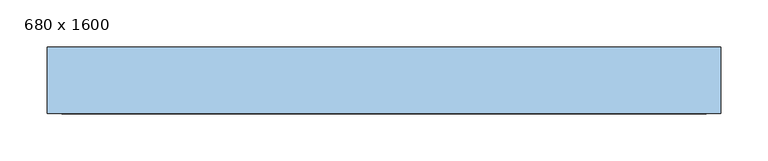
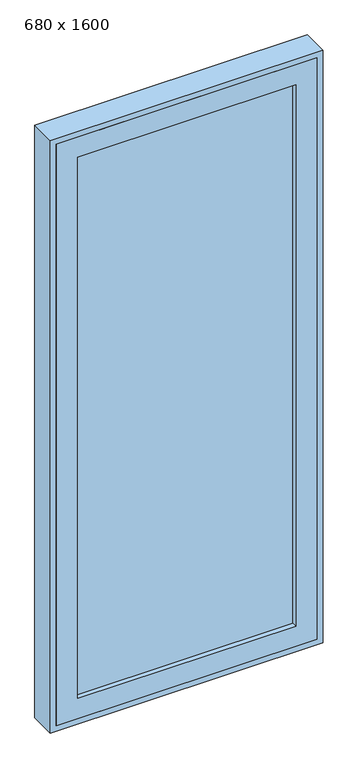
"""IFC4 building model written with IfcOpenShell, lengths in millimetres: window geometry, Aluprof_MB-79N-SI_E_Alu_Window-1sash-FIX_ENG_R-00206 : 680 x 1600."""

import ifcopenshell
import ifcopenshell.guid

model = None  # the IFC model being written
_history = None  # IfcOwnerHistory: only IFC2X3 demands one
_inside = {}  # id of a spatial element -> (the spatial element, [elements in it])
_under = {}  # id of a project, library or spatial element -> (it, [spatial elements below it])
_declared = {}  # id of a project -> (the project, [libraries it declares])
_typed = {}  # id of a type object -> (the type object, [elements of that type])
_made_of = {}  # id of a material, layer set ... -> (it, [elements and type objects made of it])


def new_model(schema):
    """Start an empty IFC model of exactly this schema.

    Asked for "IFC4X3", IfcOpenShell would pick the latest addendum, in which some entities
    have other attributes; the version numbers below select the first issue.
    IFC2X3 requires an IfcOwnerHistory on every rooted entity: one is made here for all.
    """
    global model, _history
    if schema == "IFC4X3":
        model = ifcopenshell.file(schema_version=(4, 3, 0, 0))
    else:
        model = ifcopenshell.file(schema=schema)
    _inside.clear()
    _under.clear()
    _declared.clear()
    _typed.clear()
    _made_of.clear()
    _history = None
    if model.schema == "IFC2X3":
        org = make("IfcOrganization", Name="unknown")
        user = make(
            "IfcPersonAndOrganization",
            ThePerson=make("IfcPerson", FamilyName="unknown"),
            TheOrganization=org,
        )
        app = make(
            "IfcApplication",
            ApplicationDeveloper=org,
            Version="unknown",
            ApplicationFullName="unknown",
            ApplicationIdentifier="unknown",
        )
        _history = make(
            "IfcOwnerHistory",
            OwningUser=user,
            OwningApplication=app,
            ChangeAction="ADDED",
            CreationDate=0,
        )
    return model


def make(cls, **values):
    """One entity of the class cls with the attributes given. An attribute that is None is left unset."""
    return model.create_entity(
        cls, **{name: value for name, value in values.items() if value is not None}
    )


def rooted(cls, **values):
    """An entity with a GlobalId (a new one), such as an element, a storey or a relation."""
    return make(cls, GlobalId=ifcopenshell.guid.new(), OwnerHistory=_history, **values)


def si_unit(unit_type, name, prefix=None):
    """IfcSIUnit, for example si_unit("LENGTHUNIT", "METRE", prefix="MILLI")."""
    return make("IfcSIUnit", UnitType=unit_type, Prefix=prefix, Name=name)


def assignment(units):
    """IfcUnitAssignment: the units of a project."""
    return None if units is None else make("IfcUnitAssignment", Units=units)


def point(xyz):
    """IfcCartesianPoint."""
    return None if xyz is None else make("IfcCartesianPoint", Coordinates=xyz)


def direction(xyz):
    """IfcDirection."""
    return None if xyz is None else make("IfcDirection", DirectionRatios=xyz)


def frame(location, z_axis=None, x_axis=None):
    """IfcAxis2Placement3D, a coordinate frame: its origin and axes. An axis left out is left unset."""
    return make(
        "IfcAxis2Placement3D",
        Location=point(location),
        Axis=direction(z_axis),
        RefDirection=direction(x_axis),
    )


def origin():
    """The frame at (0, 0, 0) with its axes left unset."""
    return frame((0.0, 0.0, 0.0))


def place(relative_to, where):
    """IfcLocalPlacement: puts the frame where relative to a parent placement (None: the world)."""
    return make(
        "IfcLocalPlacement", PlacementRelTo=relative_to, RelativePlacement=where
    )


def context(
    kind, dimensions, precision=None, world=None, true_north=None, identifier=None
):
    """IfcGeometricRepresentationContext, for example the 3D "Model" context."""
    return make(
        "IfcGeometricRepresentationContext",
        ContextIdentifier=identifier,
        ContextType=kind,
        CoordinateSpaceDimension=dimensions,
        Precision=precision,
        WorldCoordinateSystem=world,
        TrueNorth=true_north,
    )


def project(units=None, contexts=None):
    """IfcProject with its units and contexts."""
    return rooted(
        "IfcProject",
        Name="project",
        RepresentationContexts=contexts,
        UnitsInContext=assignment(units),
    )


def spatial(cls, under=None, at=None, **own):
    """A site, building, storey or space (cls), placed at a placement, below another one or the project."""
    s = rooted(cls, ObjectPlacement=at, **own)
    if under is not None:
        _under.setdefault(under.id(), (under, []))[1].append(s)
    return s


def polyline(points):
    """IfcPolyline through the points."""
    return make("IfcPolyline", Points=[point(p) for p in points])


def outline(outer, holes=None, kind="AREA"):
    """IfcArbitraryClosedProfileDef: a profile drawn as a closed curve; with holes, ...WithVoids."""
    if holes is None:
        return make("IfcArbitraryClosedProfileDef", ProfileType=kind, OuterCurve=outer)
    return make(
        "IfcArbitraryProfileDefWithVoids",
        ProfileType=kind,
        OuterCurve=outer,
        InnerCurves=holes,
    )


def extrude(swept, where, along, depth):
    """IfcExtrudedAreaSolid: the profile swept, set in the frame where, extruded along a direction by depth."""
    return make(
        "IfcExtrudedAreaSolid",
        SweptArea=swept,
        Position=where,
        ExtrudedDirection=direction(along),
        Depth=depth,
    )


def faces_of(points, faces, orient=None, outer=None):
    """IfcFace entities. A face is a list of loops; a loop is a list of indices into points, from 0.

    orient and outer hold one flag for each loop. By default every Orientation is true, the
    first loop of a face is its IfcFaceOuterBound and the others are IfcFaceBound.
    """
    made = []
    for i, loops in enumerate(faces):
        bounds = []
        for j, loop in enumerate(loops):
            is_outer = j == 0 if outer is None else outer[i][j]
            bounds.append(
                make(
                    "IfcFaceOuterBound" if is_outer else "IfcFaceBound",
                    Bound=make("IfcPolyLoop", Polygon=[points[k] for k in loop]),
                    Orientation=True if orient is None else orient[i][j],
                )
            )
        made.append(make("IfcFace", Bounds=bounds))
    return made


def faceted_brep(points, faces, orient=None, outer=None, voids=None):
    """IfcFacetedBrep: a solid bounded by flat faces; with voids (closed shells), ...WithVoids."""
    shared = [point(p) for p in points]
    hull = make("IfcClosedShell", CfsFaces=faces_of(shared, faces, orient, outer))
    if voids is None:
        return make("IfcFacetedBrep", Outer=hull)
    return make(
        "IfcFacetedBrepWithVoids",
        Outer=hull,
        Voids=[
            make(cls, CfsFaces=faces_of(shared, fs, o, b)) for cls, fs, o, b in voids
        ],
    )


def shape(context_of_items, identifier, shape_type, items):
    """IfcShapeRepresentation: the items that make up one representation, for example the "Body"."""
    return make(
        "IfcShapeRepresentation",
        ContextOfItems=context_of_items,
        RepresentationIdentifier=identifier,
        RepresentationType=shape_type,
        Items=items,
    )


def source(mapping_origin, context_of_items, identifier, shape_type, items):
    """IfcRepresentationMap: a shape defined once, which mapped items show again and again."""
    return make(
        "IfcRepresentationMap",
        MappingOrigin=mapping_origin,
        MappedRepresentation=shape(context_of_items, identifier, shape_type, items),
    )


def transform(
    local_origin,
    x_axis=None,
    y_axis=None,
    z_axis=None,
    scale=None,
    scale2=None,
    scale3=None,
    uniform=True,
):
    """IfcCartesianTransformationOperator3D, or its non-uniform kind. x_axis, y_axis, z_axis: its Axis1, 2, 3."""
    if uniform:
        return make(
            "IfcCartesianTransformationOperator3D",
            Axis1=direction(x_axis),
            Axis2=direction(y_axis),
            LocalOrigin=point(local_origin),
            Scale=scale,
            Axis3=direction(z_axis),
        )
    return make(
        "IfcCartesianTransformationOperator3DnonUniform",
        Axis1=direction(x_axis),
        Axis2=direction(y_axis),
        LocalOrigin=point(local_origin),
        Scale=scale,
        Axis3=direction(z_axis),
        Scale2=scale2,
        Scale3=scale3,
    )


def mapped(mapping_source, mapping_target):
    """IfcMappedItem: shows the shape of a source again, moved by a transform."""
    return make(
        "IfcMappedItem", MappingSource=mapping_source, MappingTarget=mapping_target
    )


def made_of(thing, what):
    """Note that an element or type object is made of a material, layer set ...; save() writes the relation."""
    if what is not None:
        _made_of.setdefault(what.id(), (what, []))[1].append(thing)
    return thing


def element(
    cls,
    number,
    at=None,
    inside=None,
    cuts=None,
    type_object=None,
    material=None,
    context=None,
    identifier="Body",
    shape_type=None,
    held_by="IfcProductDefinitionShape",
    body=None,
    shapes=None,
    **own,
):
    """One element of the class cls, such as IfcWall. Its Tag is "e" and its number.

    at: its placement. inside: the storey or other place that contains it. cuts: it is an
    opening in that element (IfcRelVoidsElement). A single representation is given by context,
    identifier, shape_type and body (its items); several are given by shapes. held_by: the class
    of the entity that holds the representations. save() writes the other relations.
    """
    e = rooted(cls, Tag="e%d" % number, ObjectPlacement=at, **own)
    if body is not None:
        shapes = [shape(context, identifier, shape_type, body)]
    if shapes is not None:
        e.Representation = make(held_by, Representations=shapes)
    if inside is not None:
        _inside.setdefault(inside.id(), (inside, []))[1].append(e)
    if cuts is not None:
        rooted(
            "IfcRelVoidsElement", RelatingBuildingElement=cuts, RelatedOpeningElement=e
        )
    if type_object is not None:
        _typed.setdefault(type_object.id(), (type_object, []))[1].append(e)
    return made_of(e, material)


def aggregate(whole, parts):
    """IfcRelAggregates: a whole, such as a stair, and the parts it consists of."""
    return rooted("IfcRelAggregates", RelatingObject=whole, RelatedObjects=parts)


def save(model, path):
    """Write the relations noted so far, then the file.

    IfcRelAggregates (storeys below a building ...), IfcRelContainedInSpatialStructure (elements
    in a storey), IfcRelDefinesByType, IfcRelAssociatesMaterial and IfcRelDeclares: one each for
    every whole, place, type object, material and project.
    """
    for whole, parts in _under.values():
        aggregate(whole, parts)
    for where, things in _inside.values():
        rooted(
            "IfcRelContainedInSpatialStructure",
            RelatedElements=things,
            RelatingStructure=where,
        )
    for kind, things in _typed.values():
        rooted("IfcRelDefinesByType", RelatedObjects=things, RelatingType=kind)
    for what, things in _made_of.values():
        rooted("IfcRelAssociatesMaterial", RelatedObjects=things, RelatingMaterial=what)
    for by, libraries in _declared.values():
        rooted("IfcRelDeclares", RelatingContext=by, RelatedDefinitions=libraries)
    model.write(path)


def window_680_x_1600_0a658332(model_context):
    return source(origin(), model_context, "Body", "SolidModel", [
        faceted_brep([(-284.5, 58.5, 2315.5), (-284.5, 45.0, 2315.5), (-284.5, 45.0, 826.5), (-284.5, 58.5, 826.5), (-340.0, 45.0, 2371.0), (-340.0, 115.0, 2371.0), (-340.0, 115.0, 771.0), (-340.0, 45.0, 771.0), (284.5, 45.0, 826.5), (284.5, 58.5, 826.5), (340.0, 115.0, 771.0), (340.0, 45.0, 771.0), (284.5, 45.0, 2315.5), (284.5, 58.5, 2315.5), (340.0, 115.0, 2371.0), (340.0, 45.0, 2371.0), (-300.5, 58.5, 2331.5), (300.5, 58.5, 2331.5), (300.5, 58.5, 810.5), (-300.5, 58.5, 810.5), (-300.5, 106.5, 2331.5), (-300.5, 106.5, 810.5), (300.5, 106.5, 810.5), (300.5, 106.5, 2331.5), (-281.5, 106.5, 2312.5), (281.5, 106.5, 2312.5), (281.5, 106.5, 829.5), (-281.5, 106.5, 829.5), (-281.5, 115.0, 2312.5), (-281.5, 115.0, 829.5), (281.5, 115.0, 829.5), (281.5, 115.0, 2312.5)], [[[0, 1, 2, 3]], [[4, 5, 6, 7]], [[3, 2, 8, 9]], [[7, 6, 10, 11]], [[9, 8, 12, 13]], [[11, 10, 14, 15]], [[16, 17, 18, 19], [3, 9, 13, 0]], [[13, 12, 1, 0]], [[7, 11, 15, 4], [1, 12, 8, 2]], [[15, 14, 5, 4]], [[20, 16, 19, 21]], [[21, 19, 18, 22]], [[22, 18, 17, 23]], [[21, 22, 23, 20], [24, 25, 26, 27]], [[23, 17, 16, 20]], [[28, 24, 27, 29]], [[29, 27, 26, 30]], [[30, 26, 25, 31]], [[5, 14, 10, 6], [29, 30, 31, 28]], [[31, 25, 24, 28]]]),
        extrude(outline(polyline([(300.5, 58.5), (-300.5, 58.5), (-300.5, 106.5), (300.5, 106.5), (300.5, 58.5)])), frame((0.0, 0.0, 810.5), z_axis=(0.0, 0.0, 1.0), x_axis=(1.0, 0.0, 0.0)), (0.0, 0.0, 1.0), 1521.0),
        extrude(outline(polyline([(756.0, -355.0), (756.0, 355.0), (2386.0, 355.0), (2386.0, -355.0), (756.0, -355.0)]), holes=[polyline([(2371.0, -340.0), (2371.0, 340.0), (771.0, 340.0), (771.0, -340.0), (2371.0, -340.0)])]), frame((0.0, 45.0, 0.0), z_axis=(0.0, 1.0, 0.0), x_axis=(0.0, 0.0, 1.0)), (0.0, 0.0, 1.0), 70.0),
    ])


if __name__ == "__main__":
    model = new_model("IFC4")
    model_context = context("Model", 3, world=origin())
    ifc_project = project(units=[si_unit("LENGTHUNIT", "METRE", prefix="MILLI")], contexts=[model_context])
    site = spatial("IfcSite", under=ifc_project)
    building = spatial("IfcBuilding", under=site)
    placement = place(None, origin())
    window_680_x_1600_shape = window_680_x_1600_0a658332(model_context)
    element("IfcWindow", 1, ObjectType="Aluprof_MB-79N-SI_E_Alu_Window-1sash-FIX_ENG_R-00206 : 680 x 1600", at=placement, inside=building, context=model_context, shape_type="MappedRepresentation", body=[
        mapped(window_680_x_1600_shape, transform((0.0, 0.0, 0.0), x_axis=(1.0, 0.0, 0.0), y_axis=(0.0, 1.0, 0.0), z_axis=(0.0, 0.0, 1.0))),
    ])
    save(model, "model.ifc")

# Revit data of these elements
# Type "Aluprof_MB-79N-SI_E_Alu_Window-1sash-FIX_ENG_R-00206 : 680 x 1600"
#   Type Mark = "50"
#   Water resistance = "Class E1950, EN 12208"
#   Uniclass2015Version = "v1.6"
#   Uniclass2015Reference = "Pr_30_59_98_02"
#   Uniclass2015Description = "Aluminium window units"
#   URL = "https://aluprof.eu/"
#   Resistance to wind load = "Class C5, EN 12210"
#   Product page URL = "https://aluprof.eu/architekci/katalog-dla-architektow/systemy-okienno-drzwiowe/mb-79n-si-system-okienno-drzwiowy-z-izolacja-termiczna#/materialy/ogolne-informacje"
#   Operation = "SinglePanel"
#   Opening type = "FIX"
#   NBSReference = "45-25-99/310"
#   NBSDescription = "Aluminium window units"
#   Model = "MB-79N SI"
#   Manufacturer = "ALUPROF S.A."
#   Insert type = "SI"
#   IfcExportType = "NOTDEFINED"
#   IfcExportAs = "IfcWindowType"
#   Glazing construction = "6/16/4/16/6"
#   Description = "Single fixed window"
#   Content of the recyclate in the material = "70.7%"
#   COBie.Type.WarrantyDurationParts = ""
#   COBie.Type.Name = ""
#   COBie.Type.Manufacturer = "ALUPROF SA"
#   COBie.Space.Name = ""
#   COBie.Floor.Name = ""
#   COBie.Facility.Name = ""
#   COBie.CreatedOn = ""
#   COBie.CreatedBy = "aluprof.eu"
#   COBie.Component.WarrantyStartDate = ""
#   COBie.Component.Name = "MB-79N SI"
#   Air permeability = "Class 4, EN 12207"
#   Thermal insulation = 0.6000 W/(m²·K)
#   Sash thickness = 79 mm
#   Rough Width = 710 mm
#   Rough Height = 1630 mm
#   Mounting space = 15 mm
#   Height = 1600 mm
#   Glazing area = 0.914121 m²
#   Frame thickness = 70 mm
#   Exterior wall face offset = 60 mm
#   Sill Height = 771 mm
#   Width = 680 mm
#   Warm installation [instance default] = yes
#   Schedule No. [instance default] = 1
#   IsExternal = yes
#   COBie.Type = yes
#   COBie = yes
#   GlazingMaterial = Glass_ALUPROF_Clear
#   FrameMaterial = Träfönster WSP Stockholm
#   BackfillingMaterial = ExpandingFoam_ALUPROF_Yellow
#   Wall Closure = (empty or 0)
# Element 1 (IfcWindow, "Aluprof_MB-79N-SI_E_Alu_Window-1sash-FIX_ENG_R-00206 : 680 x 1600")
#   Materials on its faces: "Träfönster WSP Stockholm", "ExpandingFoam_ALUPROF_Yellow", "Glass_ALUPROF_Clear"
# Materials
#   "Glass_ALUPROF_Clear": class "Glass", colour RGB 22 81 169, transparency 0.85, Model = "GlazingClear", Manufacturer = "ALUPROF S.A.", URL = "https://aluprof.eu/pl-en", Description = "Glazing", Cost = 0
#   "Träfönster WSP Stockholm": class "Generic", colour RGB 45 25 19, transparency 0, Cost = 0
#   "ExpandingFoam_ALUPROF_Yellow": class "Generic", colour RGB 175 175 60, transparency 0, Model = "ExpandingFoam", Manufacturer = "ALUPROF S.A.", URL = "https://aluprof.eu/pl-en", Description = "Expanding foam", Cost = 0
